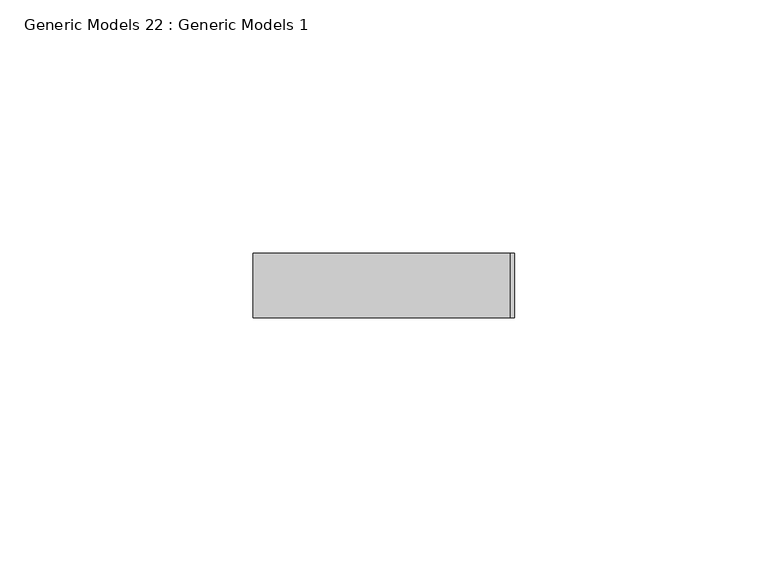
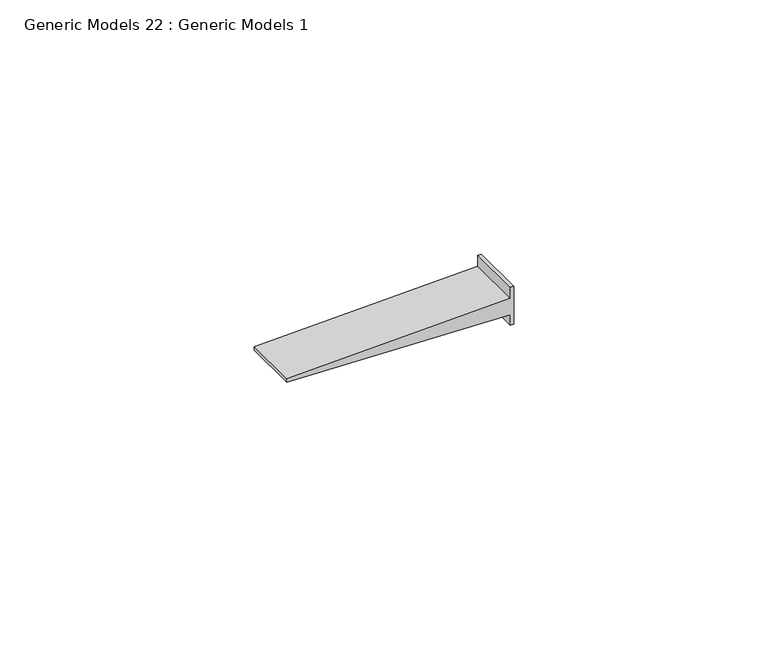
"""IFC4 building model written with IfcOpenShell, lengths in millimetres: proxy geometry, Generic Models 22 : Generic Models 1."""

from ifc_helpers import new_model, si_unit, frame, origin, place, context, project, spatial, polyline, outline, extrude, source, transform, mapped, element, save


def generic_models_22_generic_models_1_e13db24a(model_context):
    return source(origin(), model_context, "Body", "SweptSolid", [
        extrude(outline(polyline([(485.1617794, 52667.1133608), (485.1617794, 52666.3196108), (482.6119158, 52666.3196108), (481.0145267, 52615.5196108), (480.2158321, 52615.5196108), (478.618443, 52666.3196108), (476.0685794, 52666.3196108), (476.0685794, 52667.1133608), (485.1617794, 52667.1133608)])), frame((0.0, 565.15, 0.0), z_axis=(0.0, 1.0, 0.0), x_axis=(0.0, 0.0, 1.0)), (0.0, 0.0, 1.0), 12.7),
    ])


if __name__ == "__main__":
    model = new_model("IFC4")
    model_context = context("Model", 3, world=origin())
    ifc_project = project(units=[si_unit("LENGTHUNIT", "METRE", prefix="MILLI")], contexts=[model_context])
    site = spatial("IfcSite", under=ifc_project)
    building = spatial("IfcBuilding", under=site)
    placement = place(None, origin())
    generic_models_22_generic_models_1_shape = generic_models_22_generic_models_1_e13db24a(model_context)
    element("IfcBuildingElementProxy", 1, Name="Generic Models 22 : Generic Models 1", ObjectType="Generic Models 22 : Generic Models 1", at=placement, inside=building, context=model_context, shape_type="MappedRepresentation", body=[
        mapped(generic_models_22_generic_models_1_shape, transform((0.0, 0.0, 0.0), x_axis=(1.0, 0.0, 0.0), y_axis=(0.0, 1.0, 0.0), z_axis=(0.0, 0.0, 1.0))),
    ])
    save(model, "model.ifc")

# Revit data of these elements
# Element 1 (IfcBuildingElementProxy, "Generic Models 22 : Generic Models 1")
#   Materials on its faces: "ATTACH GYPSUM BOARD TO STUDS AND NOT TO TOP TRACK"
# Materials
#   "ATTACH GYPSUM BOARD TO STUDS AND NOT TO TOP TRACK": class "Generic", colour RGB 48 48 48, transparency 0, Cost = 0
